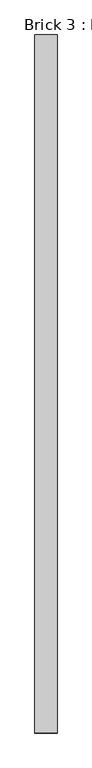
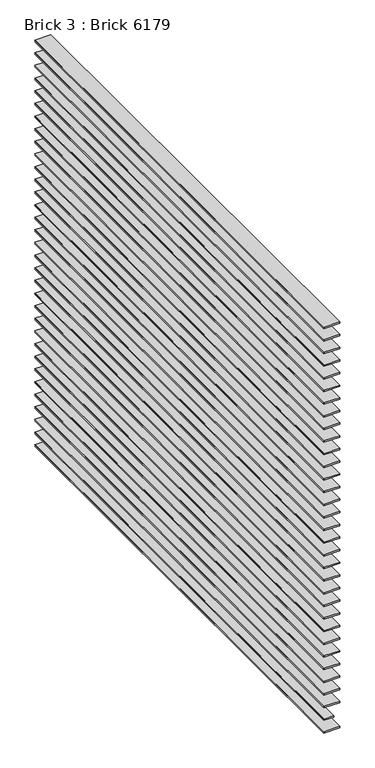
"""IFC4 building model written with IfcOpenShell, lengths in millimetres: proxy geometry, Brick 3 : Brick 6179."""

from ifc_helpers import new_model, si_unit, point, frame, frame_2d, origin, place, context, project, spatial, polyline, circle_curve, trimmed, segment, composite_curve, outline, extrude, source, transform, mapped, element, save


def brick_3_brick_6179_25ec3522(model_context):
    return source(origin(), model_context, "Body", "SweptSolid", [
        extrude(outline(composite_curve([segment(polyline([(37320.25, 10083.0612048), (37326.2029111, 10083.0612048), (37326.2029111, 10019.5612048)]), True, "CONTINUOUS"), segment(trimmed(circle_curve(frame_2d((37323.2264555, 10016.8521801)), 4.0246867), [point((37326.2029111, 10019.5612048))], [point((37320.25, 10019.5612048))], True, "CARTESIAN"), True, "CONTINUOUS"), segment(polyline([(37320.25, 10019.5612048), (37320.25, 10083.0612048)]), True, "CONTINUOUS")], self_intersect=False)), frame((0.0, 2217.3609988, 0.0), z_axis=(0.0, 1.0, 0.0), x_axis=(0.0, 0.0, 1.0)), (0.0, 0.0, 1.0), 2000.0),
        extrude(outline(composite_curve([segment(polyline([(37373.6875, 10059.8947267), (37379.6404111, 10059.8947267), (37379.6404111, 10019.5612048)]), True, "CONTINUOUS"), segment(trimmed(circle_curve(frame_2d((37376.6639555, 10016.8521801)), 4.0246867), [point((37379.6404111, 10019.5612048))], [point((37373.6875, 10019.5612048))], True, "CARTESIAN"), True, "CONTINUOUS"), segment(polyline([(37373.6875, 10019.5612048), (37373.6875, 10059.8947267)]), True, "CONTINUOUS")], self_intersect=False)), frame((0.0, 2217.3609988, 0.0), z_axis=(0.0, 1.0, 0.0), x_axis=(0.0, 0.0, 1.0)), (0.0, 0.0, 1.0), 2000.0),
        extrude(outline(composite_curve([segment(polyline([(37427.125, 10083.0612048), (37433.0779111, 10083.0612048), (37433.0779111, 10019.5612048)]), True, "CONTINUOUS"), segment(trimmed(circle_curve(frame_2d((37430.1014555, 10016.8521801)), 4.0246867), [point((37433.0779111, 10019.5612048))], [point((37427.125, 10019.5612048))], True, "CARTESIAN"), True, "CONTINUOUS"), segment(polyline([(37427.125, 10019.5612048), (37427.125, 10083.0612048)]), True, "CONTINUOUS")], self_intersect=False)), frame((0.0, 2217.3609988, 0.0), z_axis=(0.0, 1.0, 0.0), x_axis=(0.0, 0.0, 1.0)), (0.0, 0.0, 1.0), 2000.0),
        extrude(outline(composite_curve([segment(polyline([(37480.5625, 10083.0612048), (37486.5154111, 10083.0612048), (37486.5154111, 10019.5612048)]), True, "CONTINUOUS"), segment(trimmed(circle_curve(frame_2d((37483.5389555, 10016.8521801)), 4.0246867), [point((37486.5154111, 10019.5612048))], [point((37480.5625, 10019.5612048))], True, "CARTESIAN"), True, "CONTINUOUS"), segment(polyline([(37480.5625, 10019.5612048), (37480.5625, 10083.0612048)]), True, "CONTINUOUS")], self_intersect=False)), frame((0.0, 2217.3609988, 0.0), z_axis=(0.0, 1.0, 0.0), x_axis=(0.0, 0.0, 1.0)), (0.0, 0.0, 1.0), 2000.0),
        extrude(outline(composite_curve([segment(polyline([(37534.0, 10083.0612048), (37539.9529111, 10083.0612048), (37539.9529111, 10019.5612048)]), True, "CONTINUOUS"), segment(trimmed(circle_curve(frame_2d((37536.9764555, 10016.8521801)), 4.0246867), [point((37539.9529111, 10019.5612048))], [point((37534.0, 10019.5612048))], True, "CARTESIAN"), True, "CONTINUOUS"), segment(polyline([(37534.0, 10019.5612048), (37534.0, 10083.0612048)]), True, "CONTINUOUS")], self_intersect=False)), frame((0.0, 2217.3609988, 0.0), z_axis=(0.0, 1.0, 0.0), x_axis=(0.0, 0.0, 1.0)), (0.0, 0.0, 1.0), 2000.0),
        extrude(outline(composite_curve([segment(polyline([(37587.4375, 10083.0612048), (37593.3904111, 10083.0612048), (37593.3904111, 10019.5612048)]), True, "CONTINUOUS"), segment(trimmed(circle_curve(frame_2d((37590.4139555, 10016.8521801)), 4.0246867), [point((37593.3904111, 10019.5612048))], [point((37587.4375, 10019.5612048))], True, "CARTESIAN"), True, "CONTINUOUS"), segment(polyline([(37587.4375, 10019.5612048), (37587.4375, 10083.0612048)]), True, "CONTINUOUS")], self_intersect=False)), frame((0.0, 2217.3609988, 0.0), z_axis=(0.0, 1.0, 0.0), x_axis=(0.0, 0.0, 1.0)), (0.0, 0.0, 1.0), 2000.0),
        extrude(outline(composite_curve([segment(polyline([(37640.875, 10083.0612048), (37646.8279111, 10083.0612048), (37646.8279111, 10019.5612048)]), True, "CONTINUOUS"), segment(trimmed(circle_curve(frame_2d((37643.8514555, 10016.8521801)), 4.0246867), [point((37646.8279111, 10019.5612048))], [point((37640.875, 10019.5612048))], True, "CARTESIAN"), True, "CONTINUOUS"), segment(polyline([(37640.875, 10019.5612048), (37640.875, 10083.0612048)]), True, "CONTINUOUS")], self_intersect=False)), frame((0.0, 2217.3609988, 0.0), z_axis=(0.0, 1.0, 0.0), x_axis=(0.0, 0.0, 1.0)), (0.0, 0.0, 1.0), 2000.0),
        extrude(outline(composite_curve([segment(polyline([(37694.3125, 10083.0612048), (37700.2654111, 10083.0612048), (37700.2654111, 10019.5612048)]), True, "CONTINUOUS"), segment(trimmed(circle_curve(frame_2d((37697.2889555, 10016.8521801)), 4.0246867), [point((37700.2654111, 10019.5612048))], [point((37694.3125, 10019.5612048))], True, "CARTESIAN"), True, "CONTINUOUS"), segment(polyline([(37694.3125, 10019.5612048), (37694.3125, 10083.0612048)]), True, "CONTINUOUS")], self_intersect=False)), frame((0.0, 2217.3609988, 0.0), z_axis=(0.0, 1.0, 0.0), x_axis=(0.0, 0.0, 1.0)), (0.0, 0.0, 1.0), 2000.0),
        extrude(outline(composite_curve([segment(polyline([(37747.75, 10083.0612048), (37753.7029111, 10083.0612048), (37753.7029111, 10019.5612048)]), True, "CONTINUOUS"), segment(trimmed(circle_curve(frame_2d((37750.7264555, 10016.8521801)), 4.0246867), [point((37753.7029111, 10019.5612048))], [point((37747.75, 10019.5612048))], True, "CARTESIAN"), True, "CONTINUOUS"), segment(polyline([(37747.75, 10019.5612048), (37747.75, 10083.0612048)]), True, "CONTINUOUS")], self_intersect=False)), frame((0.0, 2217.3609988, 0.0), z_axis=(0.0, 1.0, 0.0), x_axis=(0.0, 0.0, 1.0)), (0.0, 0.0, 1.0), 2000.0),
        extrude(outline(composite_curve([segment(polyline([(37801.1875, 10083.0612048), (37807.1404111, 10083.0612048), (37807.1404111, 10019.5612048)]), True, "CONTINUOUS"), segment(trimmed(circle_curve(frame_2d((37804.1639555, 10016.8521801)), 4.0246867), [point((37807.1404111, 10019.5612048))], [point((37801.1875, 10019.5612048))], True, "CARTESIAN"), True, "CONTINUOUS"), segment(polyline([(37801.1875, 10019.5612048), (37801.1875, 10083.0612048)]), True, "CONTINUOUS")], self_intersect=False)), frame((0.0, 2217.3609988, 0.0), z_axis=(0.0, 1.0, 0.0), x_axis=(0.0, 0.0, 1.0)), (0.0, 0.0, 1.0), 2000.0),
        extrude(outline(composite_curve([segment(polyline([(37854.625, 10083.0612048), (37860.5779111, 10083.0612048), (37860.5779111, 10019.5612048)]), True, "CONTINUOUS"), segment(trimmed(circle_curve(frame_2d((37857.6014555, 10016.8521801)), 4.0246867), [point((37860.5779111, 10019.5612048))], [point((37854.625, 10019.5612048))], True, "CARTESIAN"), True, "CONTINUOUS"), segment(polyline([(37854.625, 10019.5612048), (37854.625, 10083.0612048)]), True, "CONTINUOUS")], self_intersect=False)), frame((0.0, 2217.3609988, 0.0), z_axis=(0.0, 1.0, 0.0), x_axis=(0.0, 0.0, 1.0)), (0.0, 0.0, 1.0), 2000.0),
        extrude(outline(composite_curve([segment(polyline([(37908.0625, 10083.0612048), (37914.0154111, 10083.0612048), (37914.0154111, 10019.5612048)]), True, "CONTINUOUS"), segment(trimmed(circle_curve(frame_2d((37911.0389555, 10016.8521801)), 4.0246867), [point((37914.0154111, 10019.5612048))], [point((37908.0625, 10019.5612048))], True, "CARTESIAN"), True, "CONTINUOUS"), segment(polyline([(37908.0625, 10019.5612048), (37908.0625, 10083.0612048)]), True, "CONTINUOUS")], self_intersect=False)), frame((0.0, 2217.3609988, 0.0), z_axis=(0.0, 1.0, 0.0), x_axis=(0.0, 0.0, 1.0)), (0.0, 0.0, 1.0), 2000.0),
        extrude(outline(composite_curve([segment(polyline([(37961.5, 10083.0612048), (37967.4529111, 10083.0612048), (37967.4529111, 10019.5612048)]), True, "CONTINUOUS"), segment(trimmed(circle_curve(frame_2d((37964.4764555, 10016.8521801)), 4.0246867), [point((37967.4529111, 10019.5612048))], [point((37961.5, 10019.5612048))], True, "CARTESIAN"), True, "CONTINUOUS"), segment(polyline([(37961.5, 10019.5612048), (37961.5, 10083.0612048)]), True, "CONTINUOUS")], self_intersect=False)), frame((0.0, 2217.3609988, 0.0), z_axis=(0.0, 1.0, 0.0), x_axis=(0.0, 0.0, 1.0)), (0.0, 0.0, 1.0), 2000.0),
        extrude(outline(composite_curve([segment(polyline([(38014.9375, 10083.0612048), (38020.8904111, 10083.0612048), (38020.8904111, 10019.5612048)]), True, "CONTINUOUS"), segment(trimmed(circle_curve(frame_2d((38017.9139555, 10016.8521801)), 4.0246867), [point((38020.8904111, 10019.5612048))], [point((38014.9375, 10019.5612048))], True, "CARTESIAN"), True, "CONTINUOUS"), segment(polyline([(38014.9375, 10019.5612048), (38014.9375, 10083.0612048)]), True, "CONTINUOUS")], self_intersect=False)), frame((0.0, 2217.3609988, 0.0), z_axis=(0.0, 1.0, 0.0), x_axis=(0.0, 0.0, 1.0)), (0.0, 0.0, 1.0), 2000.0),
        extrude(outline(composite_curve([segment(polyline([(38068.375, 10083.0612048), (38074.3279111, 10083.0612048), (38074.3279111, 10019.5612048)]), True, "CONTINUOUS"), segment(trimmed(circle_curve(frame_2d((38071.3514555, 10016.8521801)), 4.0246867), [point((38074.3279111, 10019.5612048))], [point((38068.375, 10019.5612048))], True, "CARTESIAN"), True, "CONTINUOUS"), segment(polyline([(38068.375, 10019.5612048), (38068.375, 10083.0612048)]), True, "CONTINUOUS")], self_intersect=False)), frame((0.0, 2217.3609988, 0.0), z_axis=(0.0, 1.0, 0.0), x_axis=(0.0, 0.0, 1.0)), (0.0, 0.0, 1.0), 2000.0),
        extrude(outline(composite_curve([segment(polyline([(38121.8125, 10083.0612048), (38127.7654111, 10083.0612048), (38127.7654111, 10019.5612048)]), True, "CONTINUOUS"), segment(trimmed(circle_curve(frame_2d((38124.7889555, 10016.8521801)), 4.0246867), [point((38127.7654111, 10019.5612048))], [point((38121.8125, 10019.5612048))], True, "CARTESIAN"), True, "CONTINUOUS"), segment(polyline([(38121.8125, 10019.5612048), (38121.8125, 10083.0612048)]), True, "CONTINUOUS")], self_intersect=False)), frame((0.0, 2217.3609988, 0.0), z_axis=(0.0, 1.0, 0.0), x_axis=(0.0, 0.0, 1.0)), (0.0, 0.0, 1.0), 2000.0),
        extrude(outline(composite_curve([segment(polyline([(38175.25, 10083.0612048), (38181.2029111, 10083.0612048), (38181.2029111, 10019.5612048)]), True, "CONTINUOUS"), segment(trimmed(circle_curve(frame_2d((38178.2264555, 10016.8521801)), 4.0246867), [point((38181.2029111, 10019.5612048))], [point((38175.25, 10019.5612048))], True, "CARTESIAN"), True, "CONTINUOUS"), segment(polyline([(38175.25, 10019.5612048), (38175.25, 10083.0612048)]), True, "CONTINUOUS")], self_intersect=False)), frame((0.0, 2217.3609988, 0.0), z_axis=(0.0, 1.0, 0.0), x_axis=(0.0, 0.0, 1.0)), (0.0, 0.0, 1.0), 2000.0),
        extrude(outline(composite_curve([segment(polyline([(38228.6875, 10083.0612048), (38234.6404111, 10083.0612048), (38234.6404111, 10019.5612048)]), True, "CONTINUOUS"), segment(trimmed(circle_curve(frame_2d((38231.6639555, 10016.8521801)), 4.0246867), [point((38234.6404111, 10019.5612048))], [point((38228.6875, 10019.5612048))], True, "CARTESIAN"), True, "CONTINUOUS"), segment(polyline([(38228.6875, 10019.5612048), (38228.6875, 10083.0612048)]), True, "CONTINUOUS")], self_intersect=False)), frame((0.0, 2217.3609988, 0.0), z_axis=(0.0, 1.0, 0.0), x_axis=(0.0, 0.0, 1.0)), (0.0, 0.0, 1.0), 2000.0),
        extrude(outline(composite_curve([segment(polyline([(38282.125, 10083.0612048), (38288.0779111, 10083.0612048), (38288.0779111, 10019.5612048)]), True, "CONTINUOUS"), segment(trimmed(circle_curve(frame_2d((38285.1014555, 10016.8521801)), 4.0246867), [point((38288.0779111, 10019.5612048))], [point((38282.125, 10019.5612048))], True, "CARTESIAN"), True, "CONTINUOUS"), segment(polyline([(38282.125, 10019.5612048), (38282.125, 10083.0612048)]), True, "CONTINUOUS")], self_intersect=False)), frame((0.0, 2217.3609988, 0.0), z_axis=(0.0, 1.0, 0.0), x_axis=(0.0, 0.0, 1.0)), (0.0, 0.0, 1.0), 2000.0),
        extrude(outline(composite_curve([segment(polyline([(38335.5625, 10083.0612048), (38341.5154111, 10083.0612048), (38341.5154111, 10019.5612048)]), True, "CONTINUOUS"), segment(trimmed(circle_curve(frame_2d((38338.5389555, 10016.8521801)), 4.0246867), [point((38341.5154111, 10019.5612048))], [point((38335.5625, 10019.5612048))], True, "CARTESIAN"), True, "CONTINUOUS"), segment(polyline([(38335.5625, 10019.5612048), (38335.5625, 10083.0612048)]), True, "CONTINUOUS")], self_intersect=False)), frame((0.0, 2217.3609988, 0.0), z_axis=(0.0, 1.0, 0.0), x_axis=(0.0, 0.0, 1.0)), (0.0, 0.0, 1.0), 2000.0),
        extrude(outline(composite_curve([segment(polyline([(38389.0, 10083.0612048), (38394.9529111, 10083.0612048), (38394.9529111, 10019.5612048)]), True, "CONTINUOUS"), segment(trimmed(circle_curve(frame_2d((38391.9764555, 10016.8521801)), 4.0246867), [point((38394.9529111, 10019.5612048))], [point((38389.0, 10019.5612048))], True, "CARTESIAN"), True, "CONTINUOUS"), segment(polyline([(38389.0, 10019.5612048), (38389.0, 10083.0612048)]), True, "CONTINUOUS")], self_intersect=False)), frame((0.0, 2217.3609988, 0.0), z_axis=(0.0, 1.0, 0.0), x_axis=(0.0, 0.0, 1.0)), (0.0, 0.0, 1.0), 2000.0),
        extrude(outline(composite_curve([segment(polyline([(38442.4375, 10083.0612048), (38448.3904111, 10083.0612048), (38448.3904111, 10019.5612048)]), True, "CONTINUOUS"), segment(trimmed(circle_curve(frame_2d((38445.4139555, 10016.8521801)), 4.0246867), [point((38448.3904111, 10019.5612048))], [point((38442.4375, 10019.5612048))], True, "CARTESIAN"), True, "CONTINUOUS"), segment(polyline([(38442.4375, 10019.5612048), (38442.4375, 10083.0612048)]), True, "CONTINUOUS")], self_intersect=False)), frame((0.0, 2217.3609988, 0.0), z_axis=(0.0, 1.0, 0.0), x_axis=(0.0, 0.0, 1.0)), (0.0, 0.0, 1.0), 2000.0),
        extrude(outline(composite_curve([segment(polyline([(38495.875, 10083.0612048), (38501.8279111, 10083.0612048), (38501.8279111, 10019.5612048)]), True, "CONTINUOUS"), segment(trimmed(circle_curve(frame_2d((38498.8514555, 10016.8521801)), 4.0246867), [point((38501.8279111, 10019.5612048))], [point((38495.875, 10019.5612048))], True, "CARTESIAN"), True, "CONTINUOUS"), segment(polyline([(38495.875, 10019.5612048), (38495.875, 10083.0612048)]), True, "CONTINUOUS")], self_intersect=False)), frame((0.0, 2217.3609988, 0.0), z_axis=(0.0, 1.0, 0.0), x_axis=(0.0, 0.0, 1.0)), (0.0, 0.0, 1.0), 2000.0),
        extrude(outline(composite_curve([segment(polyline([(38549.3125, 10083.0612048), (38555.2654111, 10083.0612048), (38555.2654111, 10019.5612048)]), True, "CONTINUOUS"), segment(trimmed(circle_curve(frame_2d((38552.2889555, 10016.8521801)), 4.0246867), [point((38555.2654111, 10019.5612048))], [point((38549.3125, 10019.5612048))], True, "CARTESIAN"), True, "CONTINUOUS"), segment(polyline([(38549.3125, 10019.5612048), (38549.3125, 10083.0612048)]), True, "CONTINUOUS")], self_intersect=False)), frame((0.0, 2217.3609988, 0.0), z_axis=(0.0, 1.0, 0.0), x_axis=(0.0, 0.0, 1.0)), (0.0, 0.0, 1.0), 2000.0),
        extrude(outline(composite_curve([segment(polyline([(38602.75, 10083.0612048), (38608.7029111, 10083.0612048), (38608.7029111, 10019.5612048)]), True, "CONTINUOUS"), segment(trimmed(circle_curve(frame_2d((38605.7264555, 10016.8521801)), 4.0246867), [point((38608.7029111, 10019.5612048))], [point((38602.75, 10019.5612048))], True, "CARTESIAN"), True, "CONTINUOUS"), segment(polyline([(38602.75, 10019.5612048), (38602.75, 10083.0612048)]), True, "CONTINUOUS")], self_intersect=False)), frame((0.0, 2217.3609988, 0.0), z_axis=(0.0, 1.0, 0.0), x_axis=(0.0, 0.0, 1.0)), (0.0, 0.0, 1.0), 2000.0),
        extrude(outline(composite_curve([segment(polyline([(38656.1875, 10083.0612048), (38662.1404111, 10083.0612048), (38662.1404111, 10019.5612048)]), True, "CONTINUOUS"), segment(trimmed(circle_curve(frame_2d((38659.1639555, 10016.8521801)), 4.0246867), [point((38662.1404111, 10019.5612048))], [point((38656.1875, 10019.5612048))], True, "CARTESIAN"), True, "CONTINUOUS"), segment(polyline([(38656.1875, 10019.5612048), (38656.1875, 10083.0612048)]), True, "CONTINUOUS")], self_intersect=False)), frame((0.0, 2217.3609988, 0.0), z_axis=(0.0, 1.0, 0.0), x_axis=(0.0, 0.0, 1.0)), (0.0, 0.0, 1.0), 2000.0),
        extrude(outline(composite_curve([segment(polyline([(38709.625, 10083.0612048), (38715.5779111, 10083.0612048), (38715.5779111, 10019.5612048)]), True, "CONTINUOUS"), segment(trimmed(circle_curve(frame_2d((38712.6014555, 10016.8521801)), 4.0246867), [point((38715.5779111, 10019.5612048))], [point((38709.625, 10019.5612048))], True, "CARTESIAN"), True, "CONTINUOUS"), segment(polyline([(38709.625, 10019.5612048), (38709.625, 10083.0612048)]), True, "CONTINUOUS")], self_intersect=False)), frame((0.0, 2217.3609988, 0.0), z_axis=(0.0, 1.0, 0.0), x_axis=(0.0, 0.0, 1.0)), (0.0, 0.0, 1.0), 2000.0),
        extrude(outline(composite_curve([segment(polyline([(38763.0625, 10083.0612048), (38769.0154111, 10083.0612048), (38769.0154111, 10019.5612048)]), True, "CONTINUOUS"), segment(trimmed(circle_curve(frame_2d((38766.0389555, 10016.8521801)), 4.0246867), [point((38769.0154111, 10019.5612048))], [point((38763.0625, 10019.5612048))], True, "CARTESIAN"), True, "CONTINUOUS"), segment(polyline([(38763.0625, 10019.5612048), (38763.0625, 10083.0612048)]), True, "CONTINUOUS")], self_intersect=False)), frame((0.0, 2217.3609988, 0.0), z_axis=(0.0, 1.0, 0.0), x_axis=(0.0, 0.0, 1.0)), (0.0, 0.0, 1.0), 2000.0),
        extrude(outline(composite_curve([segment(polyline([(38816.5, 10083.0612048), (38822.4529111, 10083.0612048), (38822.4529111, 10019.5612048)]), True, "CONTINUOUS"), segment(trimmed(circle_curve(frame_2d((38819.4764555, 10016.8521801)), 4.0246867), [point((38822.4529111, 10019.5612048))], [point((38816.5, 10019.5612048))], True, "CARTESIAN"), True, "CONTINUOUS"), segment(polyline([(38816.5, 10019.5612048), (38816.5, 10083.0612048)]), True, "CONTINUOUS")], self_intersect=False)), frame((0.0, 2217.3609988, 0.0), z_axis=(0.0, 1.0, 0.0), x_axis=(0.0, 0.0, 1.0)), (0.0, 0.0, 1.0), 2000.0),
        extrude(outline(composite_curve([segment(polyline([(38869.9375, 10083.0612048), (38875.8904111, 10083.0612048), (38875.8904111, 10019.5612048)]), True, "CONTINUOUS"), segment(trimmed(circle_curve(frame_2d((38872.9139555, 10016.8521801)), 4.0246867), [point((38875.8904111, 10019.5612048))], [point((38869.9375, 10019.5612048))], True, "CARTESIAN"), True, "CONTINUOUS"), segment(polyline([(38869.9375, 10019.5612048), (38869.9375, 10083.0612048)]), True, "CONTINUOUS")], self_intersect=False)), frame((0.0, 2217.3609988, 0.0), z_axis=(0.0, 1.0, 0.0), x_axis=(0.0, 0.0, 1.0)), (0.0, 0.0, 1.0), 2000.0),
        extrude(outline(composite_curve([segment(polyline([(38923.375, 10083.0612048), (38929.3279111, 10083.0612048), (38929.3279111, 10019.5612048)]), True, "CONTINUOUS"), segment(trimmed(circle_curve(frame_2d((38926.3514555, 10016.8521801)), 4.0246867), [point((38929.3279111, 10019.5612048))], [point((38923.375, 10019.5612048))], True, "CARTESIAN"), True, "CONTINUOUS"), segment(polyline([(38923.375, 10019.5612048), (38923.375, 10083.0612048)]), True, "CONTINUOUS")], self_intersect=False)), frame((0.0, 2217.3609988, 0.0), z_axis=(0.0, 1.0, 0.0), x_axis=(0.0, 0.0, 1.0)), (0.0, 0.0, 1.0), 2000.0),
        extrude(outline(composite_curve([segment(polyline([(38976.8125, 10083.0612048), (38982.7654111, 10083.0612048), (38982.7654111, 10019.5612048)]), True, "CONTINUOUS"), segment(trimmed(circle_curve(frame_2d((38979.7889555, 10016.8521801)), 4.0246867), [point((38982.7654111, 10019.5612048))], [point((38976.8125, 10019.5612048))], True, "CARTESIAN"), True, "CONTINUOUS"), segment(polyline([(38976.8125, 10019.5612048), (38976.8125, 10083.0612048)]), True, "CONTINUOUS")], self_intersect=False)), frame((0.0, 2217.3609988, 0.0), z_axis=(0.0, 1.0, 0.0), x_axis=(0.0, 0.0, 1.0)), (0.0, 0.0, 1.0), 2000.0),
        extrude(outline(composite_curve([segment(polyline([(39030.25, 10083.0612048), (39036.2029111, 10083.0612048), (39036.2029111, 10019.5612048)]), True, "CONTINUOUS"), segment(trimmed(circle_curve(frame_2d((39033.2264555, 10016.8521801)), 4.0246867), [point((39036.2029111, 10019.5612048))], [point((39030.25, 10019.5612048))], True, "CARTESIAN"), True, "CONTINUOUS"), segment(polyline([(39030.25, 10019.5612048), (39030.25, 10083.0612048)]), True, "CONTINUOUS")], self_intersect=False)), frame((0.0, 2217.3609988, 0.0), z_axis=(0.0, 1.0, 0.0), x_axis=(0.0, 0.0, 1.0)), (0.0, 0.0, 1.0), 2000.0),
    ])


if __name__ == "__main__":
    model = new_model("IFC4")
    model_context = context("Model", 3, world=origin())
    ifc_project = project(units=[si_unit("LENGTHUNIT", "METRE", prefix="MILLI")], contexts=[model_context])
    site = spatial("IfcSite", under=ifc_project)
    building = spatial("IfcBuilding", under=site)
    placement = place(None, origin())
    brick_3_brick_6179_shape = brick_3_brick_6179_25ec3522(model_context)
    element("IfcBuildingElementProxy", 1, Name="Brick 3 : Brick 6179", ObjectType="Brick 3 : Brick 6179", at=placement, inside=building, context=model_context, shape_type="MappedRepresentation", body=[
        mapped(brick_3_brick_6179_shape, transform((0.0, 0.0, 0.0), x_axis=(1.0, 0.0, 0.0), y_axis=(0.0, 1.0, 0.0), z_axis=(0.0, 0.0, 1.0))),
    ])
    save(model, "model.ifc")

# Revit data of these elements
# Type "Brick 3 : Brick 6179"
#   NameOverride = "Brick"
# Element 1 (IfcBuildingElementProxy, "Brick 3 : Brick 6179")
#   Materials on its faces: "MORTAR BED"
# Materials
#   "MORTAR BED": class "Unassigned", colour RGB 186 186 186, transparency 0, Cost = 0
